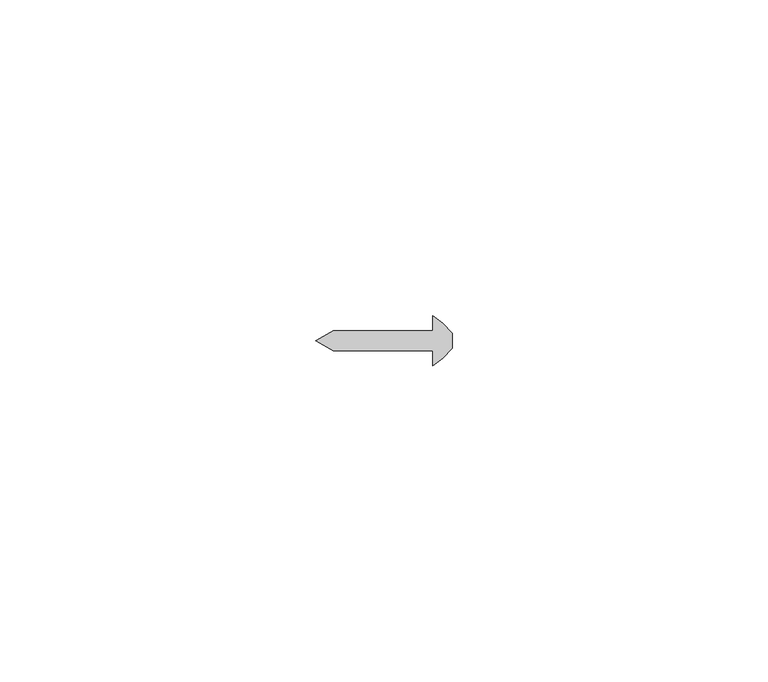
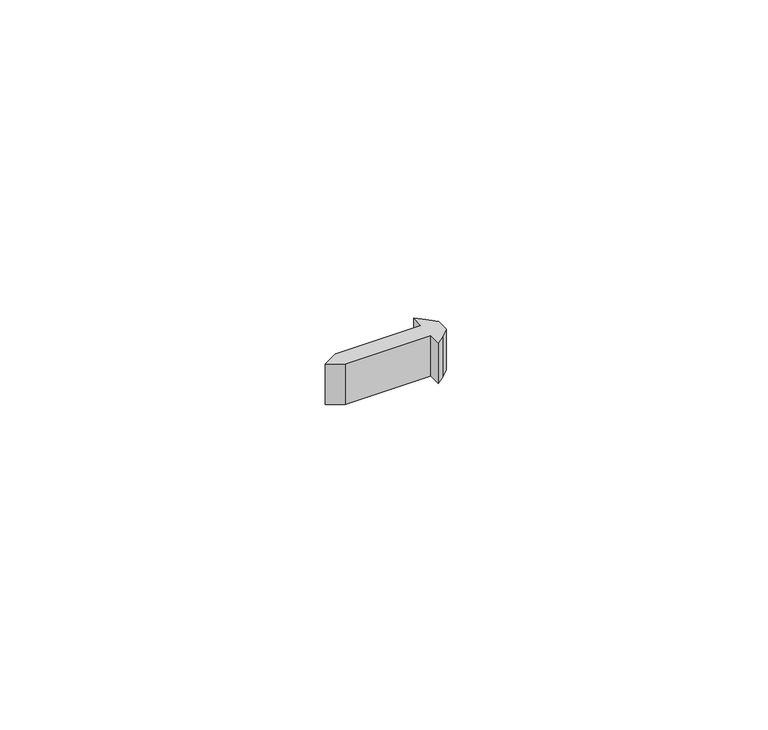
"""IFC4 building model written with IfcOpenShell, lengths in millimetres: proxy geometry, Generic Models 7:Generic Models 1:3:Generic Models 1:3 : Generic Models 7:Generic Models 1:305549:3:Generic Models 1:3:Generic Models 1:3 : Generic Models 7:Generic Models 1:305549:3 : Generic Models 7:Generic Models 1:3:Generic Models 1:3 : Generic Models 7:Generic Models 1:305549:301244:48 : Generic Models 7:Generic Models 1:3:Generic Models 1:3 : Generic Models 7:Generic Models 1:305549:3:Generic Models 1:3:Generic Models 1:3 : Generic Models 7:Generic Models 1:305549:3 : Generic Models 7:Generic Models 1:3:Generic Models 1:3 : Generic Models 7:Generic Models 1:305549:301244:308848."""

from ifc_helpers import new_model, si_unit, frame, origin, place, context, project, spatial, polyline, outline, extrude, source, transform, mapped, element, save


def generic_models_f44977b4(model_context):
    return source(origin(), model_context, "Body", "SweptSolid", [
        extrude(outline(polyline([(667631.4492239, -568268.2415363), (667615.6399684, -568268.2415363), (667612.8903378, -568266.6540363), (667615.6399684, -568265.0665363), (667631.4492239, -568265.0665363), (667631.4492239, -568262.6852863), (667632.9762819, -568263.9034819), (667634.5281721, -568265.4553721), (667634.5281721, -568267.8527006), (667632.9762819, -568269.4045908), (667631.4492239, -568270.6227863), (667631.4492239, -568268.2415363)])), frame((0.0, 0.0, 1237.45625), z_axis=(0.0, 0.0, 1.0), x_axis=(1.0, 0.0, 0.0)), (0.0, 0.0, 1.0), 7.9375),
    ])


if __name__ == "__main__":
    model = new_model("IFC4")
    model_context = context("Model", 3, world=origin())
    ifc_project = project(units=[si_unit("LENGTHUNIT", "METRE", prefix="MILLI")], contexts=[model_context])
    site = spatial("IfcSite", under=ifc_project)
    building = spatial("IfcBuilding", under=site)
    placement = place(None, origin())
    generic_models_shape = generic_models_f44977b4(model_context)
    element("IfcBuildingElementProxy", 1, Name="Generic Models 7:Generic Models 1:3:Generic Models 1:3 : Generic Models 7:Generic Models 1:305549:3:Generic Models 1:3:Generic Models 1:3 : Generic Models 7:Generic Models 1:305549:3 : Generic Models 7:Generic Models 1:3:Generic Models 1:3 : Generic Models 7:Generic Models 1:305549:301244:48 : Generic Models 7:Generic Models 1:3:Generic Models 1:3 : Generic Models 7:Generic Models 1:305549:3:Generic Models 1:3:Generic Models 1:3 : Generic Models 7:Generic Models 1:305549:3 : Generic Models 7:Generic Models 1:3:Generic Models 1:3 : Generic Models 7:Generic Models 1:305549:301244:308848", ObjectType="Generic Models 7:Generic Models 1:3:Generic Models 1:3 : Generic Models 7:Generic Models 1:305549:3:Generic Models 1:3:Generic Models 1:3 : Generic Models 7:Generic Models 1:305549:3 : Generic Models 7:Generic Models 1:3:Generic Models 1:3 : Generic Models 7:Generic Models 1:305549:301244:48 : Generic Models 7:Generic Models 1:3:Generic Models 1:3 : Generic Models 7:Generic Models 1:305549:3:Generic Models 1:3:Generic Models 1:3 : Generic Models 7:Generic Models 1:305549:3 : Generic Models 7:Generic Models 1:3:Generic Models 1:3 : Generic Models 7:Generic Models 1:305549:301244:308848", at=placement, inside=building, context=model_context, shape_type="MappedRepresentation", body=[
        mapped(generic_models_shape, transform((0.0, 0.0, 0.0), x_axis=(1.0, 0.0, 0.0), y_axis=(0.0, 1.0, 0.0), z_axis=(0.0, 0.0, 1.0))),
    ])
    save(model, "model.ifc")

# Revit data of these elements
# Type "Generic Models 7:Generic Models 1:3:Generic Models 1:3 : Generic Models 7:Generic Models 1:305549:3:Generic Models 1:3:Generic Models 1:3 : Generic Models 7:Generic Models 1:305549:3 : Generic Models 7:Generic Models 1:3:Generic Models 1:3 : Generic Models 7:Generic Models 1:305549:301244:48 : Generic Models 7:Generic Models 1:3:Generic Models 1:3 : Generic Models 7:Generic Models 1:305549:3:Generic Models 1:3:Generic Models 1:3 : Generic Models 7:Generic Models 1:305549:3 : Generic Models 7:Generic Models 1:3:Generic Models 1:3 : Generic Models 7:Generic Models 1:305549:301244:308848"
#   NameOverride = "Generic Models 7:Generic Models 1:3:Generic Models 1:3 : Generic Models 7:Generic Models 1:305549:3:Generic Models 1:3:Generic Models 1:3 : Generic Models 7:Generic Models 1:305549:3 : Generic Models 7:Generic Models 1:3:Generic Models 1:3 : Generic Models 7:Generic Models 1:305549:301244:308848"
#   ObjectTypeOverride = "Generic Models 1:3:Generic Models 1:3 : Generic Models 7:Generic Models 1:305549:3 : Generic Models 7:Generic Models 1:3:Generic Models 1:3 : Generic Models 7:Generic Models 1:305549:301244"
#   Reference = "Generic Models 1"
#   Tag = "308848"
# Element 1 (IfcBuildingElementProxy, "Generic Models 7:Generic Models 1:3:Generic Models 1:3 : Generic Models 7:Generic Models 1:305549:3:Generic Models 1:3:Generic Models 1:3 : Generic Models 7:Generic Models 1:305549:3 : Generic Models 7:Generic Models 1:3:Generic Models 1:3 : Generic Models 7:Generic Models 1:305549:301244:48 : Generic Models 7:Generic Models 1:3:Generic Models 1:3 : Generic Models 7:Generic Models 1:305549:3:Generic Models 1:3:Generic Models 1:3 : Generic Models 7:Generic Models 1:305549:3 : Generic Models 7:Generic Models 1:3:Generic Models 1:3 : Generic Models 7:Generic Models 1:305549:301244:308848")
#   Materials on its faces: "FASTENERS (T.B.D)"
# Materials
#   "FASTENERS (T.B.D)": class "Generic", colour RGB 120 120 120, transparency 0, Cost = 0
